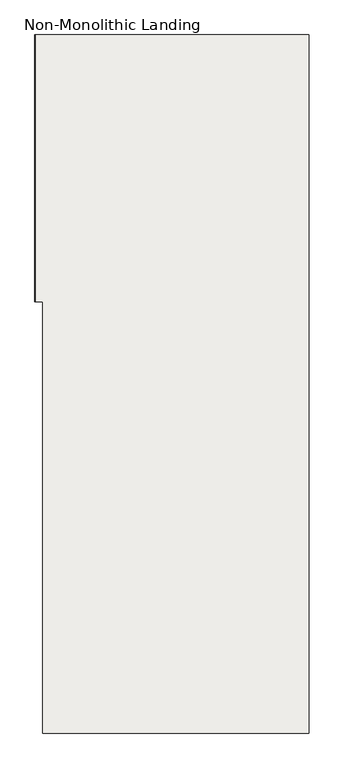
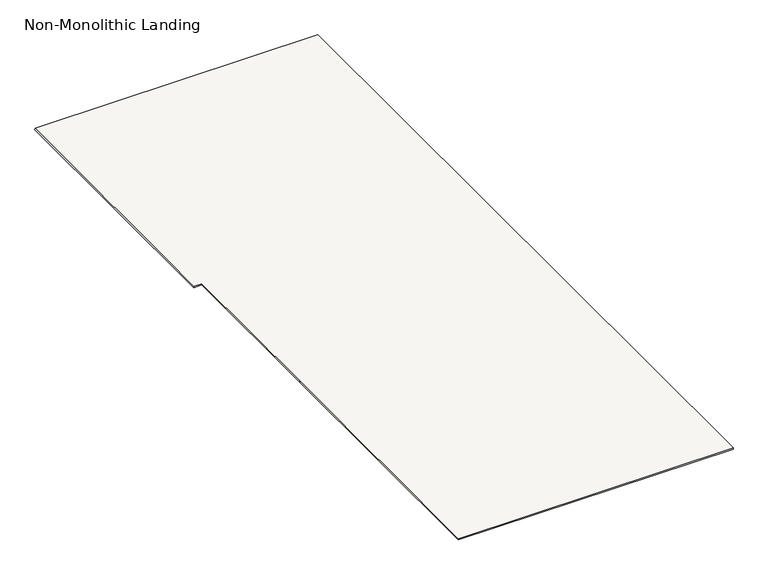
"""IFC4 building model written with IfcOpenShell, lengths in millimetres: slab geometry, Non-Monolithic Landing."""

from ifc_helpers import new_model, si_unit, origin, place, context, project, spatial, faceted_brep, source, transform, mapped, element, save


def non_monolithic_landing_33de530c(model_context):
    return source(origin(), model_context, "Body", "Brep", [
        faceted_brep([(16318.9400908, 13175.4345331, 22117.6470588), (16318.0900908, 13175.4345331, 22111.6470588), (16318.0900908, 12075.4345331, 22111.6470588), (16318.9400908, 12075.4345331, 22117.6470588), (16350.0, 10295.4345331, 22117.6470588), (17450.0, 10295.4345331, 22117.6470588), (17450.0, 13175.4345331, 22117.6470588), (16350.0, 13175.4345331, 22117.6470588), (16350.0, 12075.4345331, 22117.6470588), (16350.0, 11395.4345331, 22117.6470588), (17450.0, 13175.4345331, 22111.6470588), (17450.0, 10295.4345331, 22111.6470588), (16350.85, 10295.4345331, 22111.6470588), (16350.85, 11395.4345331, 22111.6470588), (16350.0, 11395.4345331, 22111.6470588), (16350.0, 12075.4345331, 22111.6470588), (16350.0, 13175.4345331, 22111.6470588)], [[[0, 1, 2, 3]], [[4, 5, 6, 7, 0, 3, 8, 9]], [[10, 11, 12, 13, 14, 15, 2, 1, 16]], [[9, 8, 15, 14]], [[0, 7, 16, 1]], [[7, 6, 10, 16]], [[6, 5, 11, 10]], [[5, 4, 12, 11]], [[13, 9, 14]], [[9, 13, 12, 4]], [[8, 3, 2, 15]]]),
    ])


if __name__ == "__main__":
    model = new_model("IFC4")
    model_context = context("Model", 3, world=origin())
    ifc_project = project(units=[si_unit("LENGTHUNIT", "METRE", prefix="MILLI")], contexts=[model_context])
    site = spatial("IfcSite", under=ifc_project)
    building = spatial("IfcBuilding", under=site)
    placement = place(None, origin())
    non_monolithic_landing_shape = non_monolithic_landing_33de530c(model_context)
    element("IfcSlab", 1, ObjectType="Non-Monolithic Landing", at=placement, inside=building, context=model_context, shape_type="MappedRepresentation", body=[
        mapped(non_monolithic_landing_shape, transform((0.0, 0.0, 0.0), x_axis=(1.0, 0.0, 0.0), y_axis=(0.0, 1.0, 0.0), z_axis=(0.0, 0.0, 1.0))),
    ])
    save(model, "model.ifc")

# Revit data of these elements
# Element 1 (IfcSlab, "Non-Monolithic Landing")
#   Materials on its faces: "Steel, Paint Finish, Dark Gray"
# Materials
#   "Steel, Paint Finish, Dark Gray": class "Metal", colour RGB 89 89 89, transparency 0, Description = "Steel, paint finish, dark gray, glossy", Cost = 0
